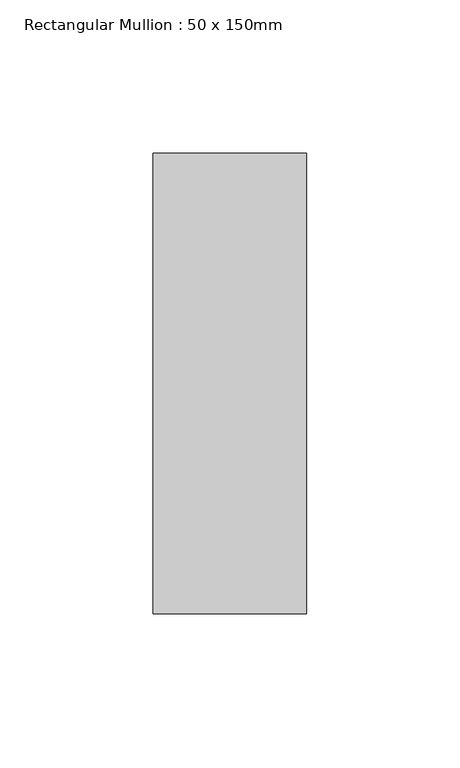
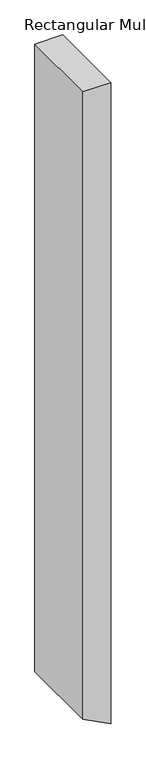
"""IFC4 building model written with IfcOpenShell, lengths in millimetres: member geometry, Rectangular Mullion : 50 x 150mm."""

from ifc_helpers import new_model, si_unit, frame, origin, place, context, project, spatial, polyline, outline, extrude, source, transform, mapped, element, save


def rectangular_mullion_50_x_150mm_3acd475a(model_context):
    return source(origin(), model_context, "Body", "SweptSolid", [
        extrude(outline(polyline([(0.0, 0.0), (0.0, -50.0), (-1194.7462362, -50.0), (-1220.7745888, 0.0), (0.0, 0.0)])), frame((0.0, -75.0, 0.0), z_axis=(0.0, 1.0, 0.0), x_axis=(0.0, 0.0, 1.0)), (0.0, 0.0, 1.0), 150.0),
    ])


if __name__ == "__main__":
    model = new_model("IFC4")
    model_context = context("Model", 3, world=origin())
    ifc_project = project(units=[si_unit("LENGTHUNIT", "METRE", prefix="MILLI")], contexts=[model_context])
    site = spatial("IfcSite", under=ifc_project)
    building = spatial("IfcBuilding", under=site)
    placement = place(None, origin())
    rectangular_mullion_50_x_150mm_shape = rectangular_mullion_50_x_150mm_3acd475a(model_context)
    element("IfcMember", 1, ObjectType="Rectangular Mullion : 50 x 150mm", at=placement, inside=building, context=model_context, shape_type="MappedRepresentation", body=[
        mapped(rectangular_mullion_50_x_150mm_shape, transform((0.0, 0.0, 0.0), x_axis=(1.0, 0.0, 0.0), y_axis=(0.0, 1.0, 0.0), z_axis=(0.0, 0.0, 1.0))),
    ])
    save(model, "model.ifc")

# Revit data of these elements
# Type "Rectangular Mullion : 50 x 150mm"
#   built-in parameter 1007304 = 0.492126 (stored number, unit not read)
#   built-in parameter 1007301 = 0.082021 (stored number, unit not read)
#   built-in parameter 1007300 = 0.082021 (stored number, unit not read)
# Element 1 (IfcMember, "Rectangular Mullion : 50 x 150mm")
#   Materials on its faces: "Aluminium"
# Materials
#   "Aluminium": class "Metal", colour RGB 247 247 247, transparency 0, Description = "Aluminium 6061", Cost = 0
